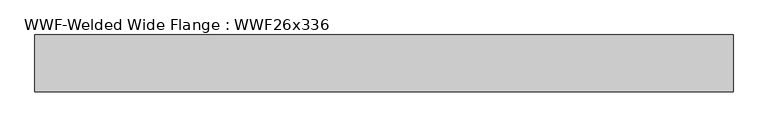
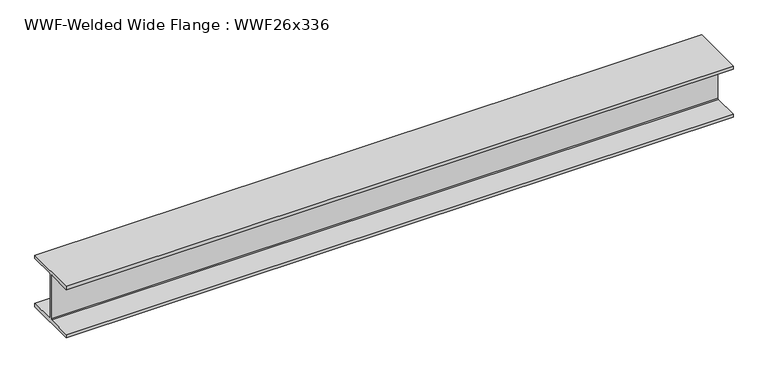
"""IFC4 building model written with IfcOpenShell, lengths in millimetres: beam geometry, WWF-Welded Wide Flange : WWF26x336."""

from ifc_helpers import new_model, si_unit, frame, origin, place, context, project, spatial, polyline, outline, extrude, source, transform, mapped, element, save


def wwf_welded_wide_flange_wwf26x336_bb5dd59e(model_context):
    return source(origin(), model_context, "Body", "SweptSolid", [
        extrude(outline(polyline([(324.993, -284.988), (324.993, -324.993), (-324.993, -324.993), (-324.993, -284.988), (-20.6375, -284.988), (-9.9949, -274.3454), (-9.9949, 274.3454), (-20.6375, 284.988), (-324.993, 284.988), (-324.993, 324.993), (324.993, 324.993), (324.993, 284.988), (20.6375, 284.988), (9.9949, 274.3454), (9.9949, -274.3454), (20.6375, -284.988), (324.993, -284.988)])), frame((-4157.4811596, 0.0, 0.0), z_axis=(1.0, 0.0, 0.0), x_axis=(0.0, 1.0, 0.0)), (0.0, 0.0, 1.0), 7985.2394153),
    ])


if __name__ == "__main__":
    model = new_model("IFC4")
    model_context = context("Model", 3, world=origin())
    ifc_project = project(units=[si_unit("LENGTHUNIT", "METRE", prefix="MILLI")], contexts=[model_context])
    site = spatial("IfcSite", under=ifc_project)
    building = spatial("IfcBuilding", under=site)
    placement = place(None, origin())
    wwf_welded_wide_flange_wwf26x336_shape = wwf_welded_wide_flange_wwf26x336_bb5dd59e(model_context)
    element("IfcBeam", 1, ObjectType="WWF-Welded Wide Flange : WWF26x336", at=placement, inside=building, context=model_context, shape_type="MappedRepresentation", body=[
        mapped(wwf_welded_wide_flange_wwf26x336_shape, transform((0.0, 0.0, 0.0), x_axis=(1.0, 0.0, 0.0), y_axis=(0.0, 1.0, 0.0), z_axis=(0.0, 0.0, 1.0))),
    ])
    save(model, "model.ifc")

# Revit data of these elements
# Type "WWF-Welded Wide Flange : WWF26x336"
#   Assembly Code = "B10"
#   Nominal d = "12"
#   W = 336
#   Length [instance default] = 1524 mm
#   bf = 649.986 mm
#   d = 649.986 mm
#   k = 20.638 mm
#   tf = 40.005 mm
#   tw = 19.99 mm
#   A = 0.0635483 m²
#   Structural Material [instance default] = Steel ASTM A572
# Element 1 (IfcBeam, "WWF-Welded Wide Flange : WWF26x336")
#   Structural Material = Metal - Steel 43-275
#   Materials on its faces: "Metal - Steel 43-275"
# Materials
#   "Steel ASTM A572": class "Metal", colour RGB 247 247 247, transparency 0, Description = "Structural steel, high strength low alloy, ASTM - A572 - 50", Cost = 0
#   "Metal - Steel 43-275": class "Metal", colour RGB 247 247 247, transparency 0, Cost = 0
